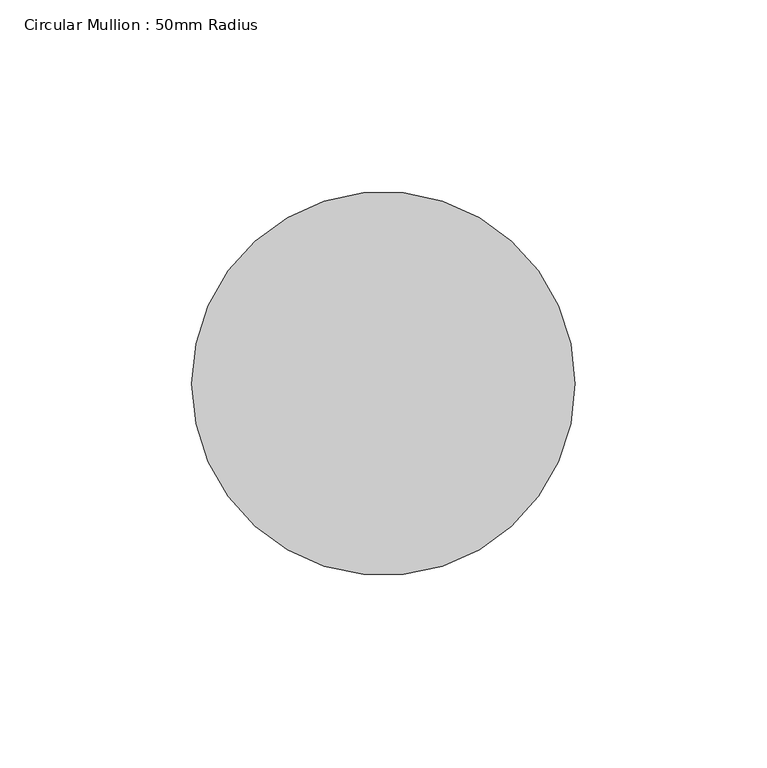
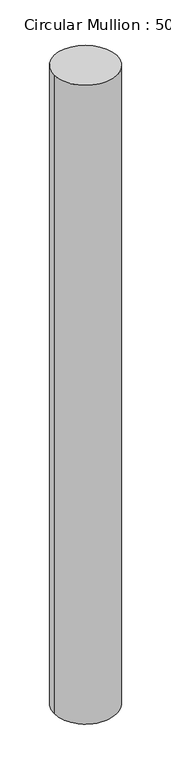
"""IFC4 building model written with IfcOpenShell, lengths in millimetres: member geometry, Circular Mullion : 50mm Radius."""

import ifcopenshell
import ifcopenshell.guid

model = None  # the IFC model being written
_history = None  # IfcOwnerHistory: only IFC2X3 demands one
_inside = {}  # id of a spatial element -> (the spatial element, [elements in it])
_under = {}  # id of a project, library or spatial element -> (it, [spatial elements below it])
_declared = {}  # id of a project -> (the project, [libraries it declares])
_typed = {}  # id of a type object -> (the type object, [elements of that type])
_made_of = {}  # id of a material, layer set ... -> (it, [elements and type objects made of it])


def new_model(schema):
    """Start an empty IFC model of exactly this schema.

    Asked for "IFC4X3", IfcOpenShell would pick the latest addendum, in which some entities
    have other attributes; the version numbers below select the first issue.
    IFC2X3 requires an IfcOwnerHistory on every rooted entity: one is made here for all.
    """
    global model, _history
    if schema == "IFC4X3":
        model = ifcopenshell.file(schema_version=(4, 3, 0, 0))
    else:
        model = ifcopenshell.file(schema=schema)
    _inside.clear()
    _under.clear()
    _declared.clear()
    _typed.clear()
    _made_of.clear()
    _history = None
    if model.schema == "IFC2X3":
        org = make("IfcOrganization", Name="unknown")
        user = make(
            "IfcPersonAndOrganization",
            ThePerson=make("IfcPerson", FamilyName="unknown"),
            TheOrganization=org,
        )
        app = make(
            "IfcApplication",
            ApplicationDeveloper=org,
            Version="unknown",
            ApplicationFullName="unknown",
            ApplicationIdentifier="unknown",
        )
        _history = make(
            "IfcOwnerHistory",
            OwningUser=user,
            OwningApplication=app,
            ChangeAction="ADDED",
            CreationDate=0,
        )
    return model


def make(cls, **values):
    """One entity of the class cls with the attributes given. An attribute that is None is left unset."""
    return model.create_entity(
        cls, **{name: value for name, value in values.items() if value is not None}
    )


def rooted(cls, **values):
    """An entity with a GlobalId (a new one), such as an element, a storey or a relation."""
    return make(cls, GlobalId=ifcopenshell.guid.new(), OwnerHistory=_history, **values)


def si_unit(unit_type, name, prefix=None):
    """IfcSIUnit, for example si_unit("LENGTHUNIT", "METRE", prefix="MILLI")."""
    return make("IfcSIUnit", UnitType=unit_type, Prefix=prefix, Name=name)


def assignment(units):
    """IfcUnitAssignment: the units of a project."""
    return None if units is None else make("IfcUnitAssignment", Units=units)


def point(xyz):
    """IfcCartesianPoint."""
    return None if xyz is None else make("IfcCartesianPoint", Coordinates=xyz)


def direction(xyz):
    """IfcDirection."""
    return None if xyz is None else make("IfcDirection", DirectionRatios=xyz)


def frame(location, z_axis=None, x_axis=None):
    """IfcAxis2Placement3D, a coordinate frame: its origin and axes. An axis left out is left unset."""
    return make(
        "IfcAxis2Placement3D",
        Location=point(location),
        Axis=direction(z_axis),
        RefDirection=direction(x_axis),
    )


def origin():
    """The frame at (0, 0, 0) with its axes left unset."""
    return frame((0.0, 0.0, 0.0))


def place(relative_to, where):
    """IfcLocalPlacement: puts the frame where relative to a parent placement (None: the world)."""
    return make(
        "IfcLocalPlacement", PlacementRelTo=relative_to, RelativePlacement=where
    )


def context(
    kind, dimensions, precision=None, world=None, true_north=None, identifier=None
):
    """IfcGeometricRepresentationContext, for example the 3D "Model" context."""
    return make(
        "IfcGeometricRepresentationContext",
        ContextIdentifier=identifier,
        ContextType=kind,
        CoordinateSpaceDimension=dimensions,
        Precision=precision,
        WorldCoordinateSystem=world,
        TrueNorth=true_north,
    )


def project(units=None, contexts=None):
    """IfcProject with its units and contexts."""
    return rooted(
        "IfcProject",
        Name="project",
        RepresentationContexts=contexts,
        UnitsInContext=assignment(units),
    )


def spatial(cls, under=None, at=None, **own):
    """A site, building, storey or space (cls), placed at a placement, below another one or the project."""
    s = rooted(cls, ObjectPlacement=at, **own)
    if under is not None:
        _under.setdefault(under.id(), (under, []))[1].append(s)
    return s


def ellipse_curve(where, semi_axis1, semi_axis2):
    """IfcEllipse in the frame where."""
    return make(
        "IfcEllipse", Position=where, SemiAxis1=semi_axis1, SemiAxis2=semi_axis2
    )


def shape(context_of_items, identifier, shape_type, items):
    """IfcShapeRepresentation: the items that make up one representation, for example the "Body"."""
    return make(
        "IfcShapeRepresentation",
        ContextOfItems=context_of_items,
        RepresentationIdentifier=identifier,
        RepresentationType=shape_type,
        Items=items,
    )


def source(mapping_origin, context_of_items, identifier, shape_type, items):
    """IfcRepresentationMap: a shape defined once, which mapped items show again and again."""
    return make(
        "IfcRepresentationMap",
        MappingOrigin=mapping_origin,
        MappedRepresentation=shape(context_of_items, identifier, shape_type, items),
    )


def transform(
    local_origin,
    x_axis=None,
    y_axis=None,
    z_axis=None,
    scale=None,
    scale2=None,
    scale3=None,
    uniform=True,
):
    """IfcCartesianTransformationOperator3D, or its non-uniform kind. x_axis, y_axis, z_axis: its Axis1, 2, 3."""
    if uniform:
        return make(
            "IfcCartesianTransformationOperator3D",
            Axis1=direction(x_axis),
            Axis2=direction(y_axis),
            LocalOrigin=point(local_origin),
            Scale=scale,
            Axis3=direction(z_axis),
        )
    return make(
        "IfcCartesianTransformationOperator3DnonUniform",
        Axis1=direction(x_axis),
        Axis2=direction(y_axis),
        LocalOrigin=point(local_origin),
        Scale=scale,
        Axis3=direction(z_axis),
        Scale2=scale2,
        Scale3=scale3,
    )


def mapped(mapping_source, mapping_target):
    """IfcMappedItem: shows the shape of a source again, moved by a transform."""
    return make(
        "IfcMappedItem", MappingSource=mapping_source, MappingTarget=mapping_target
    )


def made_of(thing, what):
    """Note that an element or type object is made of a material, layer set ...; save() writes the relation."""
    if what is not None:
        _made_of.setdefault(what.id(), (what, []))[1].append(thing)
    return thing


def element(
    cls,
    number,
    at=None,
    inside=None,
    cuts=None,
    type_object=None,
    material=None,
    context=None,
    identifier="Body",
    shape_type=None,
    held_by="IfcProductDefinitionShape",
    body=None,
    shapes=None,
    **own,
):
    """One element of the class cls, such as IfcWall. Its Tag is "e" and its number.

    at: its placement. inside: the storey or other place that contains it. cuts: it is an
    opening in that element (IfcRelVoidsElement). A single representation is given by context,
    identifier, shape_type and body (its items); several are given by shapes. held_by: the class
    of the entity that holds the representations. save() writes the other relations.
    """
    e = rooted(cls, Tag="e%d" % number, ObjectPlacement=at, **own)
    if body is not None:
        shapes = [shape(context, identifier, shape_type, body)]
    if shapes is not None:
        e.Representation = make(held_by, Representations=shapes)
    if inside is not None:
        _inside.setdefault(inside.id(), (inside, []))[1].append(e)
    if cuts is not None:
        rooted(
            "IfcRelVoidsElement", RelatingBuildingElement=cuts, RelatedOpeningElement=e
        )
    if type_object is not None:
        _typed.setdefault(type_object.id(), (type_object, []))[1].append(e)
    return made_of(e, material)


def aggregate(whole, parts):
    """IfcRelAggregates: a whole, such as a stair, and the parts it consists of."""
    return rooted("IfcRelAggregates", RelatingObject=whole, RelatedObjects=parts)


def save(model, path):
    """Write the relations noted so far, then the file.

    IfcRelAggregates (storeys below a building ...), IfcRelContainedInSpatialStructure (elements
    in a storey), IfcRelDefinesByType, IfcRelAssociatesMaterial and IfcRelDeclares: one each for
    every whole, place, type object, material and project.
    """
    for whole, parts in _under.values():
        aggregate(whole, parts)
    for where, things in _inside.values():
        rooted(
            "IfcRelContainedInSpatialStructure",
            RelatedElements=things,
            RelatingStructure=where,
        )
    for kind, things in _typed.values():
        rooted("IfcRelDefinesByType", RelatedObjects=things, RelatingType=kind)
    for what, things in _made_of.values():
        rooted("IfcRelAssociatesMaterial", RelatedObjects=things, RelatingMaterial=what)
    for by, libraries in _declared.values():
        rooted("IfcRelDeclares", RelatingContext=by, RelatedDefinitions=libraries)
    model.write(path)


def plane_surface(at):
    """IfcPlane: the flat surface through the origin of the frame at, square to its z axis."""
    return make("IfcPlane", Position=at)


def cylinder_surface(at, radius):
    """IfcCylindricalSurface: all points at the distance radius from the z axis of the frame at."""
    return make("IfcCylindricalSurface", Position=at, Radius=radius)


def advanced_brep(points, edges, surfaces, faces):
    """IfcAdvancedBrep: a solid bounded by faces that lie on surfaces and meet in shared edges.

    An edge is (start, end): straight between two places in points (the first is 0);
    or (start, end, curve); or (start, end, curve, False) where it runs against its curve.
    A face is (place in surfaces, loops), or (place, loops, False) where it looks against
    its surface's normal. A loop lists edges by number (the first is 1), with a minus sign
    where the edge is run from its end to its start. The first loop is the outer one.
    """
    corners = [point(p) for p in points]
    vertices = [make("IfcVertexPoint", VertexGeometry=c) for c in corners]
    made = []
    for start, end, *more in edges:
        made.append(
            make(
                "IfcEdgeCurve",
                EdgeStart=vertices[start],
                EdgeEnd=vertices[end],
                EdgeGeometry=more[0] if more else make("IfcPolyline", Points=[corners[start], corners[end]]),
                SameSense=more[1] if len(more) > 1 else True,
            )
        )
    hull = []
    for where, loops, *sense in faces:
        bounds = []
        for j, loop in enumerate(loops):
            ring = [make("IfcOrientedEdge", EdgeElement=made[abs(k) - 1], Orientation=k > 0) for k in loop]
            bounds.append(
                make(
                    "IfcFaceOuterBound" if j == 0 else "IfcFaceBound",
                    Bound=make("IfcEdgeLoop", EdgeList=ring),
                    Orientation=True,
                )
            )
        hull.append(make("IfcAdvancedFace", Bounds=bounds, FaceSurface=surfaces[where], SameSense=sense[0] if sense else True))
    return make("IfcAdvancedBrep", Outer=make("IfcClosedShell", CfsFaces=hull))


def circular_mullion_50mm_radius_763ddcfb(model_context):
    return source(origin(), model_context, "Body", "AdvancedBrep", [
        advanced_brep(
        [(-100.0, 0.0, 1.529687), (0.0, 0.0, 0.0), (0.0, 0.0, -1072.7298784), (-100.0, 0.0, -1074.3301609)],
        [
            (0, 1, ellipse_curve(frame((-50.0, 0.0, 0.7648435), z_axis=(-0.015291460283911403, -0.021755258862351877, -0.9996463774526559), x_axis=(-0.5748423856693377, -0.8178319580404051, 0.02659172889794555)), 50.0176874, 50.0)),
            (1, 2),
            (2, 3, ellipse_curve(frame((-50.0, 0.0, -1073.5300196), z_axis=(-0.015996631815302805, -0.022758510933958427, 0.9996130040924012), x_axis=(0.5748231944609306, 0.8178046545846791, 0.027818016632478175)), 50.0193573, 50.0)),
            (3, 0),
            (1, 0, ellipse_curve(frame((-50.0, 0.0, 0.7648435), z_axis=(-0.015291460283911403, -0.021755258862351877, -0.9996463774526559), x_axis=(-0.5748423856693377, -0.8178319580404051, 0.02659172889794555)), 50.0176874, 50.0)),
            (3, 2, ellipse_curve(frame((-50.0, 0.0, -1073.5300196), z_axis=(-0.015996631815302805, -0.022758510933958427, 0.9996130040924012), x_axis=(0.5748231944609306, 0.8178046545846791, 0.027818016632478175)), 50.0193573, 50.0)),
        ],
        [
            cylinder_surface(frame((-50.0, 0.0, 0.0), z_axis=(0.0, 0.0, 1.0), x_axis=(1.0, 0.0, 0.0)), 50.0),
            plane_surface(frame((-249.3633613, 175.27394, 0.0), z_axis=(0.015291460283911403, 0.021755258862351877, 0.9996463774526559), x_axis=(0.5748423856693362, 0.8178319580404056, -0.02659172889795584))),
            plane_surface(frame((-249.3633613, 175.27394, -1072.7298784), z_axis=(0.0159966318153028, 0.022758510933958424, -0.999613004092401), x_axis=(0.5748231944609303, 0.8178046545846789, 0.027818016632489506))),
        ],
        [
            (0, [[1, 2, 3, 4]]),
            (0, [[5, -4, 6, -2]]),
            (1, [[-1, -5]]),
            (2, [[-6, -3]]),
        ],
    ),
    ])


if __name__ == "__main__":
    model = new_model("IFC4")
    model_context = context("Model", 3, world=origin())
    ifc_project = project(units=[si_unit("LENGTHUNIT", "METRE", prefix="MILLI")], contexts=[model_context])
    site = spatial("IfcSite", under=ifc_project)
    building = spatial("IfcBuilding", under=site)
    placement = place(None, origin())
    circular_mullion_50mm_radius_shape = circular_mullion_50mm_radius_763ddcfb(model_context)
    element("IfcMember", 1, ObjectType="Circular Mullion : 50mm Radius", at=placement, inside=building, context=model_context, shape_type="MappedRepresentation", body=[
        mapped(circular_mullion_50mm_radius_shape, transform((0.0, 0.0, 0.0), x_axis=(1.0, 0.0, 0.0), y_axis=(0.0, 1.0, 0.0), z_axis=(0.0, 0.0, 1.0))),
    ])
    save(model, "model.ifc")

# Revit data of these elements
# Type "Circular Mullion : 50mm Radius"
#   built-in parameter 1007350 = 0.164042 (stored number, unit not read)
# Element 1 (IfcMember, "Circular Mullion : 50mm Radius")
#   Materials on its faces: "Aluminium"
# Materials
#   "Aluminium": class "Metal", colour RGB 247 247 247, transparency 0, Description = "Aluminium 6061", Cost = 0
